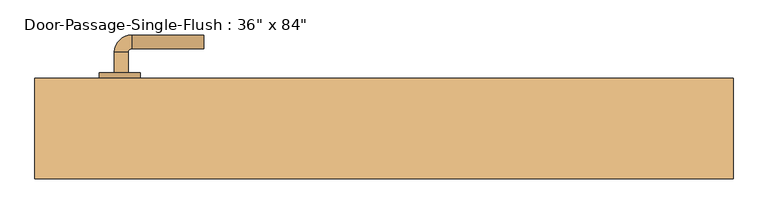
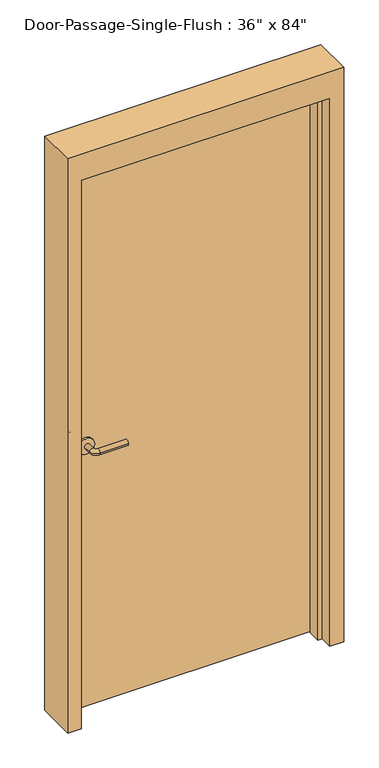
"""IFC4 building model written with IfcOpenShell, lengths in millimetres: door geometry."""

from ifc_helpers import new_model, si_unit, point, frame, frame_2d, origin, origin_with_axes, place, context, project, spatial, polyline, circle_curve, ellipse_curve, trimmed, segment, composite_curve, outline, extrude, faceted_brep, source, transform, mapped, element, save
from ifc_brep_helpers import plane_surface, cylinder_surface, revolved_surface, advanced_brep


def door_87fe937e(model_context):
    return source(origin(), model_context, "Body", "SolidModel", [
        advanced_brep(
        [(-392.190625, 25.3375, 1016.0), (-372.190625, 25.3375, 1016.0), (-372.190625, -4.6625, 1016.0), (-392.190625, -4.6625, 1016.0), (-367.190625, -9.6625, 1016.0), (-367.190625, -29.6625, 1016.0), (-262.190625, -29.6625, 1016.0), (-262.190625, -9.6625, 1016.0)],
        [
            (0, 1, circle_curve(frame((-382.190625, 25.3375, 1016.0), z_axis=(0.0, 1.0, 0.0), x_axis=(1.0, 0.0, 0.0)), 10.0)),
            (1, 0, circle_curve(frame((-382.190625, 25.3375, 1016.0), z_axis=(0.0, 1.0, 0.0), x_axis=(1.0, 0.0, 0.0)), 10.0)),
            (1, 2),
            (2, 3, circle_curve(frame((-382.190625, -4.6625, 1016.0), z_axis=(0.0, 1.0, 0.0), x_axis=(1.0, 0.0, 0.0)), 10.0)),
            (3, 0),
            (3, 2, circle_curve(frame((-382.190625, -4.6625, 1016.0), z_axis=(0.0, 1.0, 0.0), x_axis=(1.0, 0.0, 0.0)), 10.0)),
            (4, 5, circle_curve(frame((-367.190625, -19.6625, 1016.0), z_axis=(-1.0, 0.0, 0.0), x_axis=(0.0, 1.0, 0.0)), 10.0)),
            (5, 3, circle_curve(frame((-367.190625, -4.6625, 1016.0), z_axis=(0.0, 0.0, -1.0), x_axis=(-1.0, 0.0, 0.0)), 25.0)),
            (2, 4, circle_curve(frame((-367.190625, -4.6625, 1016.0), z_axis=(0.0, 0.0, 1.0), x_axis=(-1.0, 0.0, 0.0)), 5.0)),
            (5, 4, circle_curve(frame((-367.190625, -19.6625, 1016.0), z_axis=(-1.0, 0.0, 0.0), x_axis=(0.0, 1.0, 0.0)), 10.0)),
            (6, 7, circle_curve(frame((-262.190625, -19.6625, 1016.0), z_axis=(1.0, 0.0, 0.0), x_axis=(0.0, 1.0, 0.0)), 10.0)),
            (7, 6, circle_curve(frame((-262.190625, -19.6625, 1016.0), z_axis=(1.0, 0.0, 0.0), x_axis=(0.0, 1.0, 0.0)), 10.0)),
            (4, 7),
            (6, 5),
        ],
        [
            plane_surface(frame((-382.190625, 25.3375, 1016.0), z_axis=(0.0, 1.0, 0.0), x_axis=(0.0, 0.0, 1.0))),
            cylinder_surface(frame((-382.190625, 25.3375, 1016.0), z_axis=(0.0, 1.0, 0.0), x_axis=(1.0, 0.0, 0.0)), 10.0),
            revolved_surface(trimmed(ellipse_curve(frame((-382.190625, -4.6625, 1016.0), z_axis=(0.0, -1.0, 0.0), x_axis=(1.0, 0.0, 0.0)), 10.0, 10.0), [point((-392.190625, -4.6625, 1016.0))], [point((-372.190625, -4.6625, 1016.0))], True, "CARTESIAN"), (-367.190625, -4.6625, 1016.0), (0.0, 0.0, -1.0)),
            revolved_surface(trimmed(ellipse_curve(frame((-382.190625, -4.6625, 1016.0), z_axis=(0.0, -1.0, 0.0), x_axis=(1.0, 0.0, 0.0)), 10.0, 10.0), [point((-372.190625, -4.6625, 1016.0))], [point((-392.190625, -4.6625, 1016.0))], True, "CARTESIAN"), (-367.190625, -4.6625, 1016.0), (0.0, 0.0, -1.0)),
            plane_surface(frame((-262.190625, -19.6625, 1016.0), z_axis=(1.0, 0.0, 0.0), x_axis=(0.0, 0.0, 1.0))),
            cylinder_surface(frame((-367.190625, -19.6625, 1016.0), z_axis=(-1.0, 0.0, 0.0), x_axis=(0.0, 1.0, 0.0)), 10.0),
        ],
        [
            (0, [[1, 2]]),
            (1, [[3, 4, 5, -2]]),
            (1, [[-5, 6, -3, -1]]),
            (2, [[7, 8, -4, 9]]),
            (3, [[10, -9, -6, -8]]),
            (4, [[11, 12]]),
            (5, [[13, -11, 14, -7]]),
            (5, [[-14, -12, -13, -10]]),
        ],
    ),
        extrude(outline(composite_curve([segment(trimmed(circle_curve(frame_2d((1016.0, -384.690625)), 30.0), [point((1016.0, -414.690625))], [point((1016.0, -354.690625))], False, "CARTESIAN"), True, "CONTINUOUS"), segment(trimmed(circle_curve(frame_2d((1016.0, -384.690625)), 30.0), [point((1016.0, -354.690625))], [point((1016.0, -414.690625))], False, "CARTESIAN"), True, "CONTINUOUS")], self_intersect=False)), frame((0.0, 25.3375, 0.0), z_axis=(0.0, 1.0, 0.0), x_axis=(0.0, 0.0, 1.0)), (0.0, 0.0, 1.0), 8.0),
        advanced_brep(
        [(-392.190625, 85.7875, 1016.0), (-372.190625, 85.7875, 1016.0), (-392.190625, 115.7875, 1016.0), (-372.190625, 115.7875, 1016.0), (-367.190625, 120.7875, 1016.0), (-367.190625, 140.7875, 1016.0), (-262.190625, 140.7875, 1016.0), (-262.190625, 120.7875, 1016.0)],
        [
            (0, 1, circle_curve(frame((-382.190625, 85.7875, 1016.0), z_axis=(0.0, -1.0, 0.0), x_axis=(1.0, 0.0, 0.0)), 10.0)),
            (1, 0, circle_curve(frame((-382.190625, 85.7875, 1016.0), z_axis=(0.0, -1.0, 0.0), x_axis=(1.0, 0.0, 0.0)), 10.0)),
            (0, 2),
            (2, 3, circle_curve(frame((-382.190625, 115.7875, 1016.0), z_axis=(0.0, -1.0, 0.0), x_axis=(1.0, 0.0, 0.0)), 10.0)),
            (3, 1),
            (3, 2, circle_curve(frame((-382.190625, 115.7875, 1016.0), z_axis=(0.0, -1.0, 0.0), x_axis=(1.0, 0.0, 0.0)), 10.0)),
            (4, 3, circle_curve(frame((-367.190625, 115.7875, 1016.0), z_axis=(0.0, 0.0, 1.0), x_axis=(-1.0, 0.0, 0.0)), 5.0)),
            (2, 5, circle_curve(frame((-367.190625, 115.7875, 1016.0), z_axis=(0.0, 0.0, -1.0), x_axis=(-1.0, 0.0, 0.0)), 25.0)),
            (5, 4, circle_curve(frame((-367.190625, 130.7875, 1016.0), z_axis=(-1.0, 0.0, 0.0), x_axis=(0.0, -1.0, 0.0)), 10.0)),
            (4, 5, circle_curve(frame((-367.190625, 130.7875, 1016.0), z_axis=(-1.0, 0.0, 0.0), x_axis=(0.0, -1.0, 0.0)), 10.0)),
            (6, 7, circle_curve(frame((-262.190625, 130.7875, 1016.0), z_axis=(1.0, 0.0, 0.0), x_axis=(0.0, -1.0, 0.0)), 10.0)),
            (7, 6, circle_curve(frame((-262.190625, 130.7875, 1016.0), z_axis=(1.0, 0.0, 0.0), x_axis=(0.0, -1.0, 0.0)), 10.0)),
            (5, 6),
            (7, 4),
        ],
        [
            plane_surface(frame((-382.190625, 85.7875, 1016.0), z_axis=(0.0, -1.0, 0.0), x_axis=(0.0, 0.0, 1.0))),
            cylinder_surface(frame((-382.190625, 85.7875, 1016.0), z_axis=(0.0, -1.0, 0.0), x_axis=(1.0, 0.0, 0.0)), 10.0),
            revolved_surface(trimmed(ellipse_curve(frame((-382.190625, 115.7875, 1016.0), z_axis=(0.0, -1.0, 0.0), x_axis=(1.0, 0.0, 0.0)), 10.0, 10.0), [point((-392.190625, 115.7875, 1016.0))], [point((-372.190625, 115.7875, 1016.0))], True, "CARTESIAN"), (-367.190625, 115.7875, 1016.0), (0.0, 0.0, -1.0)),
            revolved_surface(trimmed(ellipse_curve(frame((-382.190625, 115.7875, 1016.0), z_axis=(0.0, -1.0, 0.0), x_axis=(1.0, 0.0, 0.0)), 10.0, 10.0), [point((-372.190625, 115.7875, 1016.0))], [point((-392.190625, 115.7875, 1016.0))], True, "CARTESIAN"), (-367.190625, 115.7875, 1016.0), (0.0, 0.0, -1.0)),
            plane_surface(frame((-262.190625, 130.7875, 1016.0), z_axis=(1.0, 0.0, 0.0), x_axis=(0.0, 0.0, 1.0))),
            cylinder_surface(frame((-367.190625, 130.7875, 1016.0), z_axis=(-1.0, 0.0, 0.0), x_axis=(0.0, -1.0, 0.0)), 10.0),
        ],
        [
            (0, [[1, 2]]),
            (1, [[-1, 3, 4, 5]]),
            (1, [[-2, -5, 6, -3]]),
            (2, [[7, -4, 8, 9]]),
            (3, [[-8, -6, -7, 10]]),
            (4, [[11, 12]]),
            (5, [[-9, 13, -12, 14]]),
            (5, [[-10, -14, -11, -13]]),
        ],
    ),
        extrude(outline(composite_curve([segment(trimmed(circle_curve(frame_2d((1016.0, -384.690625)), 30.0), [point((1016.0, -414.690625))], [point((1016.0, -354.690625))], False, "CARTESIAN"), True, "CONTINUOUS"), segment(trimmed(circle_curve(frame_2d((1016.0, -384.690625)), 30.0), [point((1016.0, -354.690625))], [point((1016.0, -414.690625))], False, "CARTESIAN"), True, "CONTINUOUS")], self_intersect=False)), frame((0.0, 77.7875, 0.0), z_axis=(0.0, 1.0, 0.0), x_axis=(0.0, 0.0, 1.0)), (0.0, 0.0, 1.0), 8.0),
        faceted_brep([(457.2, 28.575, 0.0), (457.2, 77.7875, 0.0), (508.0, 77.7875, 0.0), (508.0, -68.2625, 0.0), (457.2, -68.2625, 0.0), (457.2, -19.05, 0.0), (441.325, -19.05, 0.0), (441.325, 28.575, 0.0), (457.2, 28.575, 2133.6), (457.2, 77.7875, 2133.6), (-457.2, 77.7875, 2133.6), (-457.2, 77.7875, 0.0), (-508.0, 77.7875, 0.0), (-508.0, 77.7875, 2235.2), (508.0, 77.7875, 2235.2), (508.0, -68.2625, 2235.2), (-508.0, -68.2625, 2235.2), (-508.0, -68.2625, 0.0), (-457.2, -68.2625, 0.0), (-457.2, -68.2625, 2133.6), (457.2, -68.2625, 2133.6), (457.2, -19.05, 2133.6), (-457.2, -19.05, 2133.6), (-457.2, -19.05, 0.0), (-441.325, -19.05, 0.0), (-441.325, -19.05, 2117.725), (441.325, -19.05, 2117.725), (441.325, 28.575, 2117.725), (-441.325, 28.575, 2117.725), (-441.325, 28.575, 0.0), (-457.2, 28.575, 0.0), (-457.2, 28.575, 2133.6)], [[[0, 1, 2, 3, 4, 5, 6, 7]], [[1, 0, 8, 9]], [[2, 1, 9, 10, 11, 12, 13, 14]], [[3, 2, 14, 15]], [[4, 3, 15, 16, 17, 18, 19, 20]], [[5, 4, 20, 21]], [[6, 5, 21, 22, 23, 24, 25, 26]], [[7, 6, 26, 27]], [[0, 7, 27, 28, 29, 30, 31, 8]], [[9, 8, 31, 10]], [[20, 19, 22, 21]], [[26, 25, 28, 27]], [[12, 11, 30, 29, 24, 23, 18, 17]], [[11, 10, 31, 30]], [[13, 12, 17, 16]], [[19, 18, 23, 22]], [[25, 24, 29, 28]], [[15, 14, 13, 16]]]),
        extrude(outline(polyline([(457.2, 33.3375), (-457.2, 33.3375), (-457.2, 77.7875), (457.2, 77.7875), (457.2, 33.3375)])), origin_with_axes(), (0.0, 0.0, 1.0), 2133.6),
    ])


if __name__ == "__main__":
    model = new_model("IFC4")
    model_context = context("Model", 3, world=origin())
    ifc_project = project(units=[si_unit("LENGTHUNIT", "METRE", prefix="MILLI")], contexts=[model_context])
    site = spatial("IfcSite", under=ifc_project)
    building = spatial("IfcBuilding", under=site)
    placement = place(None, origin())
    door_shape = door_87fe937e(model_context)
    element("IfcDoor", 1, ObjectType="Door-Passage-Single-Flush : 36\" x 84\"", at=placement, inside=building, context=model_context, shape_type="MappedRepresentation", body=[
        mapped(door_shape, transform((0.0, 0.0, 0.0), x_axis=(1.0, 0.0, 0.0), y_axis=(0.0, 1.0, 0.0), z_axis=(0.0, 0.0, 1.0))),
    ])
    save(model, "model.ifc")

# Revit data of these elements
# Type "Door-Passage-Single-Flush : 36\" x 84\""
#   Type Mark = "1"
#   Assembly Code = "B2030200"
#   Analytic Construction = "Wooden"
#   Thickness = 0' - 1 3/4"
#   Thermal Resistance (R) = 2.5876 (h·ft²·°F)/BTU
#   Swing Angle [instance default] = 90.00°
#   Strike Height = 3' - 4"
#   Rough Width [instance default] = 3' - 4"
#   Rough Height [instance default] = 7' - 4"
#   MF Opening Height [instance default] = 0' - 4"
#   MF Opening Width [instance default] = 0' - 4"
#   Inset Calculate [instance default] = 0' - 4"
#   Masonry Inset [instance default] = 0' - 1"
#   Height = 7' - 0"
#   Width = 3' - 0"
#   Heat Transfer Coefficient (U) = 0.3865 BTU/(h·ft²·°F)
#   Masonry Frame Depth = 0' - 5 3/4"
#   Define Thermal Properties by = 1
#   Masonry Frame [instance default] = yes
#   Function = 1
#   Dry Wall Frame [instance default] = no
#   Panel Material = Wood - Birch
#   Frame Material = Metal - Paint Finish - Grey
#   Door Handle Material = Aluminum
#   Visual Light Transmittance = 0
#   Solar Heat Gain Coefficient = 0
#   Wall Closure = (empty or 0)
# Element 1 (IfcDoor, "Door-Passage-Single-Flush : 36\" x 84\"")
#   Materials on its faces: "Aluminum", "Metal - Paint Finish - Grey", "Wood - Birch"
# Materials
#   "Wood - Birch": class "Wood", colour RGB 166 116 52, transparency 0, Cost = 0
#   "Metal - Paint Finish - Grey": class "Paint", colour RGB 104 104 104, transparency 0, Cost = 0
#   "Aluminum": class "Metal", colour RGB 247 247 247, transparency 0, Description = "Aluminum 6061", Cost = 0
